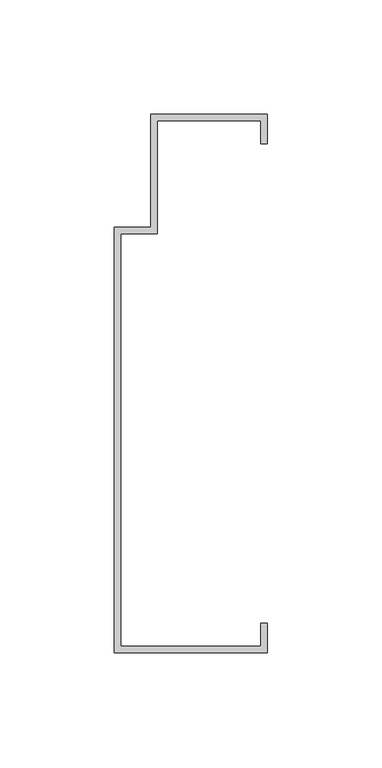
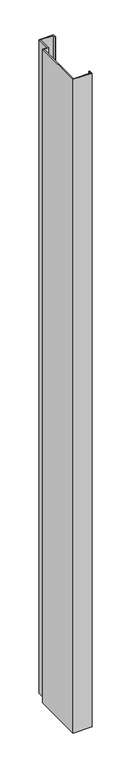
"""IFC4 building model written with IfcOpenShell, lengths in millimetres: proxy geometry, Generic Models 7:Generic Models 1:337419:Generic Models 1:337419 : Generic Models 7:Generic Models 1:337419:48 : Generic Models 7:Generic Models 1:337419:Generic Models 1:337419 : Generic Models 7:Generic Models 1:337419:301336."""

import ifcopenshell
import ifcopenshell.guid

model = None  # the IFC model being written
_history = None  # IfcOwnerHistory: only IFC2X3 demands one
_inside = {}  # id of a spatial element -> (the spatial element, [elements in it])
_under = {}  # id of a project, library or spatial element -> (it, [spatial elements below it])
_declared = {}  # id of a project -> (the project, [libraries it declares])
_typed = {}  # id of a type object -> (the type object, [elements of that type])
_made_of = {}  # id of a material, layer set ... -> (it, [elements and type objects made of it])


def new_model(schema):
    """Start an empty IFC model of exactly this schema.

    Asked for "IFC4X3", IfcOpenShell would pick the latest addendum, in which some entities
    have other attributes; the version numbers below select the first issue.
    IFC2X3 requires an IfcOwnerHistory on every rooted entity: one is made here for all.
    """
    global model, _history
    if schema == "IFC4X3":
        model = ifcopenshell.file(schema_version=(4, 3, 0, 0))
    else:
        model = ifcopenshell.file(schema=schema)
    _inside.clear()
    _under.clear()
    _declared.clear()
    _typed.clear()
    _made_of.clear()
    _history = None
    if model.schema == "IFC2X3":
        org = make("IfcOrganization", Name="unknown")
        user = make(
            "IfcPersonAndOrganization",
            ThePerson=make("IfcPerson", FamilyName="unknown"),
            TheOrganization=org,
        )
        app = make(
            "IfcApplication",
            ApplicationDeveloper=org,
            Version="unknown",
            ApplicationFullName="unknown",
            ApplicationIdentifier="unknown",
        )
        _history = make(
            "IfcOwnerHistory",
            OwningUser=user,
            OwningApplication=app,
            ChangeAction="ADDED",
            CreationDate=0,
        )
    return model


def make(cls, **values):
    """One entity of the class cls with the attributes given. An attribute that is None is left unset."""
    return model.create_entity(
        cls, **{name: value for name, value in values.items() if value is not None}
    )


def rooted(cls, **values):
    """An entity with a GlobalId (a new one), such as an element, a storey or a relation."""
    return make(cls, GlobalId=ifcopenshell.guid.new(), OwnerHistory=_history, **values)


def si_unit(unit_type, name, prefix=None):
    """IfcSIUnit, for example si_unit("LENGTHUNIT", "METRE", prefix="MILLI")."""
    return make("IfcSIUnit", UnitType=unit_type, Prefix=prefix, Name=name)


def assignment(units):
    """IfcUnitAssignment: the units of a project."""
    return None if units is None else make("IfcUnitAssignment", Units=units)


def point(xyz):
    """IfcCartesianPoint."""
    return None if xyz is None else make("IfcCartesianPoint", Coordinates=xyz)


def direction(xyz):
    """IfcDirection."""
    return None if xyz is None else make("IfcDirection", DirectionRatios=xyz)


def frame(location, z_axis=None, x_axis=None):
    """IfcAxis2Placement3D, a coordinate frame: its origin and axes. An axis left out is left unset."""
    return make(
        "IfcAxis2Placement3D",
        Location=point(location),
        Axis=direction(z_axis),
        RefDirection=direction(x_axis),
    )


def origin():
    """The frame at (0, 0, 0) with its axes left unset."""
    return frame((0.0, 0.0, 0.0))


def origin_with_axes():
    """The frame at (0, 0, 0) with the z axis (0, 0, 1) and the x axis (1, 0, 0) written out."""
    return frame((0.0, 0.0, 0.0), z_axis=(0.0, 0.0, 1.0), x_axis=(1.0, 0.0, 0.0))


def place(relative_to, where):
    """IfcLocalPlacement: puts the frame where relative to a parent placement (None: the world)."""
    return make(
        "IfcLocalPlacement", PlacementRelTo=relative_to, RelativePlacement=where
    )


def context(
    kind, dimensions, precision=None, world=None, true_north=None, identifier=None
):
    """IfcGeometricRepresentationContext, for example the 3D "Model" context."""
    return make(
        "IfcGeometricRepresentationContext",
        ContextIdentifier=identifier,
        ContextType=kind,
        CoordinateSpaceDimension=dimensions,
        Precision=precision,
        WorldCoordinateSystem=world,
        TrueNorth=true_north,
    )


def project(units=None, contexts=None):
    """IfcProject with its units and contexts."""
    return rooted(
        "IfcProject",
        Name="project",
        RepresentationContexts=contexts,
        UnitsInContext=assignment(units),
    )


def spatial(cls, under=None, at=None, **own):
    """A site, building, storey or space (cls), placed at a placement, below another one or the project."""
    s = rooted(cls, ObjectPlacement=at, **own)
    if under is not None:
        _under.setdefault(under.id(), (under, []))[1].append(s)
    return s


def polyline(points):
    """IfcPolyline through the points."""
    return make("IfcPolyline", Points=[point(p) for p in points])


def outline(outer, holes=None, kind="AREA"):
    """IfcArbitraryClosedProfileDef: a profile drawn as a closed curve; with holes, ...WithVoids."""
    if holes is None:
        return make("IfcArbitraryClosedProfileDef", ProfileType=kind, OuterCurve=outer)
    return make(
        "IfcArbitraryProfileDefWithVoids",
        ProfileType=kind,
        OuterCurve=outer,
        InnerCurves=holes,
    )


def extrude(swept, where, along, depth):
    """IfcExtrudedAreaSolid: the profile swept, set in the frame where, extruded along a direction by depth."""
    return make(
        "IfcExtrudedAreaSolid",
        SweptArea=swept,
        Position=where,
        ExtrudedDirection=direction(along),
        Depth=depth,
    )


def shape(context_of_items, identifier, shape_type, items):
    """IfcShapeRepresentation: the items that make up one representation, for example the "Body"."""
    return make(
        "IfcShapeRepresentation",
        ContextOfItems=context_of_items,
        RepresentationIdentifier=identifier,
        RepresentationType=shape_type,
        Items=items,
    )


def source(mapping_origin, context_of_items, identifier, shape_type, items):
    """IfcRepresentationMap: a shape defined once, which mapped items show again and again."""
    return make(
        "IfcRepresentationMap",
        MappingOrigin=mapping_origin,
        MappedRepresentation=shape(context_of_items, identifier, shape_type, items),
    )


def transform(
    local_origin,
    x_axis=None,
    y_axis=None,
    z_axis=None,
    scale=None,
    scale2=None,
    scale3=None,
    uniform=True,
):
    """IfcCartesianTransformationOperator3D, or its non-uniform kind. x_axis, y_axis, z_axis: its Axis1, 2, 3."""
    if uniform:
        return make(
            "IfcCartesianTransformationOperator3D",
            Axis1=direction(x_axis),
            Axis2=direction(y_axis),
            LocalOrigin=point(local_origin),
            Scale=scale,
            Axis3=direction(z_axis),
        )
    return make(
        "IfcCartesianTransformationOperator3DnonUniform",
        Axis1=direction(x_axis),
        Axis2=direction(y_axis),
        LocalOrigin=point(local_origin),
        Scale=scale,
        Axis3=direction(z_axis),
        Scale2=scale2,
        Scale3=scale3,
    )


def mapped(mapping_source, mapping_target):
    """IfcMappedItem: shows the shape of a source again, moved by a transform."""
    return make(
        "IfcMappedItem", MappingSource=mapping_source, MappingTarget=mapping_target
    )


def made_of(thing, what):
    """Note that an element or type object is made of a material, layer set ...; save() writes the relation."""
    if what is not None:
        _made_of.setdefault(what.id(), (what, []))[1].append(thing)
    return thing


def element(
    cls,
    number,
    at=None,
    inside=None,
    cuts=None,
    type_object=None,
    material=None,
    context=None,
    identifier="Body",
    shape_type=None,
    held_by="IfcProductDefinitionShape",
    body=None,
    shapes=None,
    **own,
):
    """One element of the class cls, such as IfcWall. Its Tag is "e" and its number.

    at: its placement. inside: the storey or other place that contains it. cuts: it is an
    opening in that element (IfcRelVoidsElement). A single representation is given by context,
    identifier, shape_type and body (its items); several are given by shapes. held_by: the class
    of the entity that holds the representations. save() writes the other relations.
    """
    e = rooted(cls, Tag="e%d" % number, ObjectPlacement=at, **own)
    if body is not None:
        shapes = [shape(context, identifier, shape_type, body)]
    if shapes is not None:
        e.Representation = make(held_by, Representations=shapes)
    if inside is not None:
        _inside.setdefault(inside.id(), (inside, []))[1].append(e)
    if cuts is not None:
        rooted(
            "IfcRelVoidsElement", RelatingBuildingElement=cuts, RelatedOpeningElement=e
        )
    if type_object is not None:
        _typed.setdefault(type_object.id(), (type_object, []))[1].append(e)
    return made_of(e, material)


def aggregate(whole, parts):
    """IfcRelAggregates: a whole, such as a stair, and the parts it consists of."""
    return rooted("IfcRelAggregates", RelatingObject=whole, RelatedObjects=parts)


def save(model, path):
    """Write the relations noted so far, then the file.

    IfcRelAggregates (storeys below a building ...), IfcRelContainedInSpatialStructure (elements
    in a storey), IfcRelDefinesByType, IfcRelAssociatesMaterial and IfcRelDeclares: one each for
    every whole, place, type object, material and project.
    """
    for whole, parts in _under.values():
        aggregate(whole, parts)
    for where, things in _inside.values():
        rooted(
            "IfcRelContainedInSpatialStructure",
            RelatedElements=things,
            RelatingStructure=where,
        )
    for kind, things in _typed.values():
        rooted("IfcRelDefinesByType", RelatedObjects=things, RelatingType=kind)
    for what, things in _made_of.values():
        rooted("IfcRelAssociatesMaterial", RelatedObjects=things, RelatingMaterial=what)
    for by, libraries in _declared.values():
        rooted("IfcRelDeclares", RelatingContext=by, RelatedDefinitions=libraries)
    model.write(path)


def generic_models_25deb305(model_context):
    return source(origin(), model_context, "Body", "SweptSolid", [
        extrude(outline(polyline([(593798.4117242, -536557.2913358), (593798.4117242, -536569.9913358), (593795.6335992, -536569.9913358), (593795.6335992, -536560.0694608), (593750.3898492, -536560.0694608), (593750.3898492, -536609.2819608), (593734.5148492, -536609.2819608), (593734.5148492, -536789.4632108), (593795.6335992, -536789.4632108), (593795.6335992, -536779.5413358), (593798.4117242, -536779.5413358), (593798.4117242, -536792.2413358), (593731.7367242, -536792.2413358), (593731.7367242, -536606.5038358), (593747.6117242, -536606.5038358), (593747.6117242, -536557.2913358), (593798.4117242, -536557.2913358)])), origin_with_axes(), (0.0, 0.0, 1.0), 2438.4),
    ])


if __name__ == "__main__":
    model = new_model("IFC4")
    model_context = context("Model", 3, world=origin())
    ifc_project = project(units=[si_unit("LENGTHUNIT", "METRE", prefix="MILLI")], contexts=[model_context])
    site = spatial("IfcSite", under=ifc_project)
    building = spatial("IfcBuilding", under=site)
    placement = place(None, origin())
    generic_models_shape = generic_models_25deb305(model_context)
    element("IfcBuildingElementProxy", 1, Name="Generic Models 7:Generic Models 1:337419:Generic Models 1:337419 : Generic Models 7:Generic Models 1:337419:48 : Generic Models 7:Generic Models 1:337419:Generic Models 1:337419 : Generic Models 7:Generic Models 1:337419:301336", ObjectType="Generic Models 7:Generic Models 1:337419:Generic Models 1:337419 : Generic Models 7:Generic Models 1:337419:48 : Generic Models 7:Generic Models 1:337419:Generic Models 1:337419 : Generic Models 7:Generic Models 1:337419:301336", at=placement, inside=building, context=model_context, shape_type="MappedRepresentation", body=[
        mapped(generic_models_shape, transform((0.0, 0.0, 0.0), x_axis=(1.0, 0.0, 0.0), y_axis=(0.0, 1.0, 0.0), z_axis=(0.0, 0.0, 1.0))),
    ])
    save(model, "model.ifc")

# Revit data of these elements
# Type "Generic Models 7:Generic Models 1:337419:Generic Models 1:337419 : Generic Models 7:Generic Models 1:337419:48 : Generic Models 7:Generic Models 1:337419:Generic Models 1:337419 : Generic Models 7:Generic Models 1:337419:301336"
#   NameOverride = "Generic Models 7:Generic Models 1:337419:Generic Models 1:337419 : Generic Models 7:Generic Models 1:337419:301336"
#   ObjectTypeOverride = "Generic Models 1:337419 : Generic Models 7:Generic Models 1:337419"
#   Reference = "Generic Models 1"
#   Tag = "301336"
# Element 1 (IfcBuildingElementProxy, "Generic Models 7:Generic Models 1:337419:Generic Models 1:337419 : Generic Models 7:Generic Models 1:337419:48 : Generic Models 7:Generic Models 1:337419:Generic Models 1:337419 : Generic Models 7:Generic Models 1:337419:301336")
#   Materials on its faces: "HOLLOW METAL FRAME - SEE DOOR SCHEDULE"
# Materials
#   "HOLLOW METAL FRAME - SEE DOOR SCHEDULE": class "Unassigned", colour RGB 210 209 208, transparency 0, Keynote = "M05121300.02", Cost = 0
